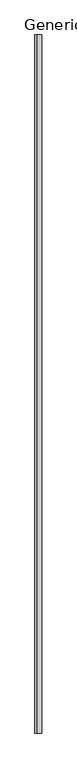
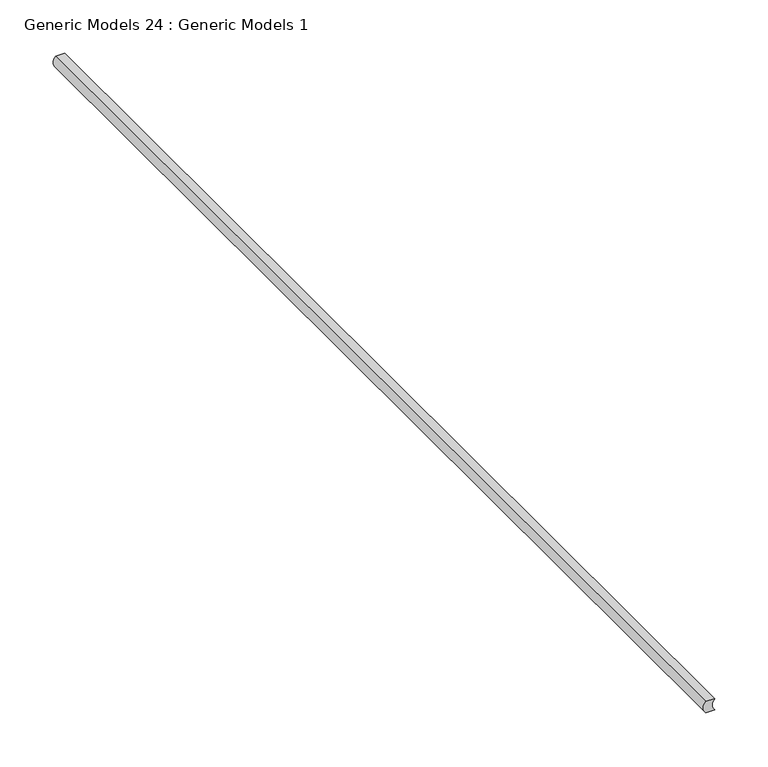
"""IFC4 building model written with IfcOpenShell, lengths in millimetres: proxy geometry, Generic Models 24 : Generic Models 1."""

from ifc_helpers import new_model, si_unit, point, frame, frame_2d, origin, place, context, project, spatial, polyline, circle_curve, trimmed, segment, composite_curve, outline, extrude, source, transform, mapped, element, save


def generic_models_24_generic_models_1_a9595ea3(model_context):
    return source(origin(), model_context, "Body", "SweptSolid", [
        extrude(outline(composite_curve([segment(trimmed(circle_curve(frame_2d((2451.1, 49805.704481)), 8.620055), [point((2444.75, 49799.875))], [point((2457.45, 49799.875))], True, "CARTESIAN"), True, "CONTINUOUS"), segment(polyline([(2457.45, 49799.875), (2457.45, 49790.35)]), True, "CONTINUOUS"), segment(trimmed(circle_curve(frame_2d((2451.1, 49796.179481)), 8.620055), [point((2457.45, 49790.35))], [point((2444.75, 49790.35))], False, "CARTESIAN"), True, "CONTINUOUS"), segment(polyline([(2444.75, 49790.35), (2444.75, 49799.875)]), True, "CONTINUOUS")], self_intersect=False)), frame((0.0, 0.0, 0.0), z_axis=(0.0, 1.0, 0.0), x_axis=(0.0, 0.0, 1.0)), (0.0, 0.0, 1.0), 1219.2),
    ])


if __name__ == "__main__":
    model = new_model("IFC4")
    model_context = context("Model", 3, world=origin())
    ifc_project = project(units=[si_unit("LENGTHUNIT", "METRE", prefix="MILLI")], contexts=[model_context])
    site = spatial("IfcSite", under=ifc_project)
    building = spatial("IfcBuilding", under=site)
    placement = place(None, origin())
    generic_models_24_generic_models_1_shape = generic_models_24_generic_models_1_a9595ea3(model_context)
    element("IfcBuildingElementProxy", 1, Name="Generic Models 24 : Generic Models 1", ObjectType="Generic Models 24 : Generic Models 1", at=placement, inside=building, context=model_context, shape_type="MappedRepresentation", body=[
        mapped(generic_models_24_generic_models_1_shape, transform((0.0, 0.0, 0.0), x_axis=(1.0, 0.0, 0.0), y_axis=(0.0, 1.0, 0.0), z_axis=(0.0, 0.0, 1.0))),
    ])
    save(model, "model.ifc")

# Revit data of these elements
# Element 1 (IfcBuildingElementProxy, "Generic Models 24 : Generic Models 1")
#   Materials on its faces: "ACOUSTICAL SEALANT"
# Materials
#   "ACOUSTICAL SEALANT": class "Unassigned", colour RGB 120 120 120, transparency 0, Cost = 0
